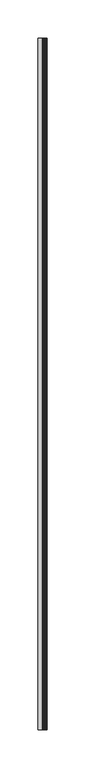
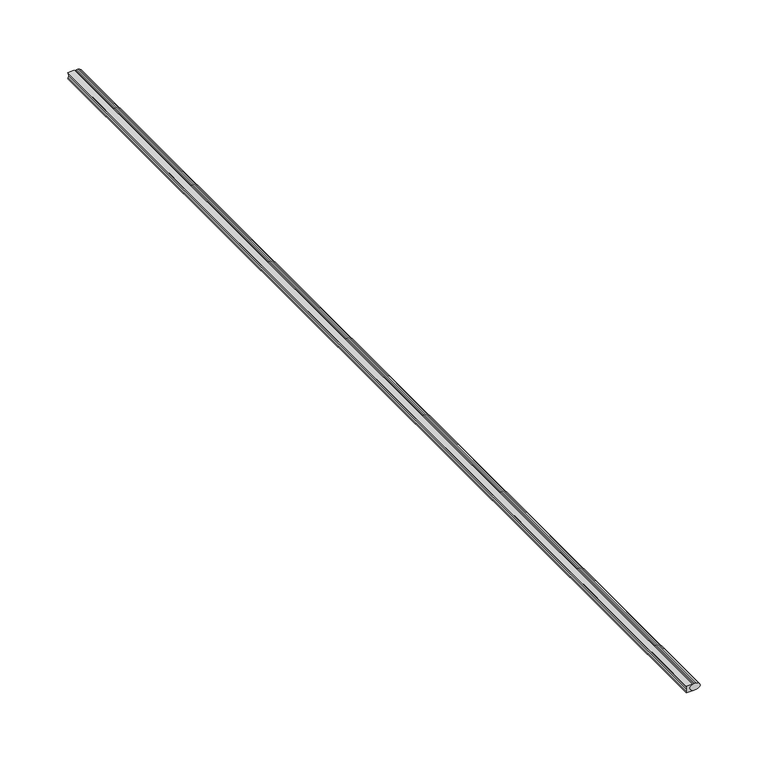
"""IFC4 building model written with IfcOpenShell, lengths in millimetres: proxy geometry, Generic Models 7:Generic Models 1:1:Generic Models 1:1 : Generic Models 7:Generic Models 1:337419:54 : Generic Models 7:Generic Models 1:1:Generic Models 1:1 : Generic Models 7:Generic Models 1:337419:306201."""

from ifc_helpers import new_model, si_unit, frame, origin, place, context, project, spatial, polyline, outline, extrude, source, transform, mapped, element, save


def generic_models_7e0ec5bf(model_context):
    return source(origin(), model_context, "Body", "SweptSolid", [
        extrude(outline(polyline([(3909.2187499, 560286.8641878), (3909.2187499, 560281.5242239), (3908.3399053, 560281.8676658), (3906.3294999, 560282.1531201), (3904.3190944, 560281.8676658), (3903.4402499, 560281.5242239), (3903.4402499, 560286.8641878), (3904.2435877, 560285.4143605), (3905.3732472, 560284.527834), (3906.6525036, 560284.343297), (3907.8812291, 560284.8896187), (3908.8672009, 560286.0813321), (3909.2187499, 560286.8641878)])), frame((0.0, -546570.8498979, 0.0), z_axis=(0.0, 1.0, 0.0), x_axis=(0.0, 0.0, 1.0)), (0.0, 0.0, 1.0), 910.0612812),
        extrude(outline(polyline([(3909.1463103, 560289.9794668), (3909.2187499, 560289.0150888), (3909.1463103, 560288.0507109), (3908.5884065, 560286.312962), (3907.5830985, 560285.1104024), (3906.3294999, 560284.6812138), (3905.0759013, 560285.1104024), (3904.0705932, 560286.312962), (3903.5126894, 560288.0507109), (3903.4402499, 560289.0150888), (3903.5126894, 560289.9794668), (3904.0705932, 560291.7172157), (3905.0759013, 560292.9197753), (3906.3294999, 560293.3489638), (3907.5830985, 560292.9197753), (3908.5884065, 560291.7172157), (3909.1463103, 560289.9794668)])), frame((0.0, -546570.8498979, 0.0), z_axis=(0.0, 1.0, 0.0), x_axis=(0.0, 0.0, 1.0)), (0.0, 0.0, 1.0), 910.0612812),
    ])


if __name__ == "__main__":
    model = new_model("IFC4")
    model_context = context("Model", 3, world=origin())
    ifc_project = project(units=[si_unit("LENGTHUNIT", "METRE", prefix="MILLI")], contexts=[model_context])
    site = spatial("IfcSite", under=ifc_project)
    building = spatial("IfcBuilding", under=site)
    placement = place(None, origin())
    generic_models_shape = generic_models_7e0ec5bf(model_context)
    element("IfcBuildingElementProxy", 1, Name="Generic Models 7:Generic Models 1:1:Generic Models 1:1 : Generic Models 7:Generic Models 1:337419:54 : Generic Models 7:Generic Models 1:1:Generic Models 1:1 : Generic Models 7:Generic Models 1:337419:306201", ObjectType="Generic Models 7:Generic Models 1:1:Generic Models 1:1 : Generic Models 7:Generic Models 1:337419:54 : Generic Models 7:Generic Models 1:1:Generic Models 1:1 : Generic Models 7:Generic Models 1:337419:306201", at=placement, inside=building, context=model_context, shape_type="MappedRepresentation", body=[
        mapped(generic_models_shape, transform((0.0, 0.0, 0.0), x_axis=(1.0, 0.0, 0.0), y_axis=(0.0, 1.0, 0.0), z_axis=(0.0, 0.0, 1.0))),
    ])
    save(model, "model.ifc")

# Revit data of these elements
# Type "Generic Models 7:Generic Models 1:1:Generic Models 1:1 : Generic Models 7:Generic Models 1:337419:54 : Generic Models 7:Generic Models 1:1:Generic Models 1:1 : Generic Models 7:Generic Models 1:337419:306201"
#   NameOverride = "Generic Models 7:Generic Models 1:1:Generic Models 1:1 : Generic Models 7:Generic Models 1:337419:306201"
#   ObjectTypeOverride = "Generic Models 1:1 : Generic Models 7:Generic Models 1:337419"
#   Reference = "Generic Models 1"
#   Tag = "306201"
# Element 1 (IfcBuildingElementProxy, "Generic Models 7:Generic Models 1:1:Generic Models 1:1 : Generic Models 7:Generic Models 1:337419:54 : Generic Models 7:Generic Models 1:1:Generic Models 1:1 : Generic Models 7:Generic Models 1:337419:306201")
#   Materials on its faces: "SEMI-RIGID EPOXY SEALANT W/ BACKROD (REMOVE TEMP. JOINT FORM)"
# Materials
#   "SEMI-RIGID EPOXY SEALANT W/ BACKROD (REMOVE TEMP. JOINT FORM)": class "Unassigned", colour RGB 120 120 120, transparency 0, Cost = 0
